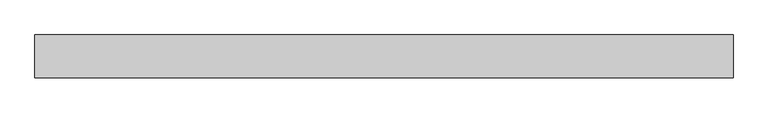
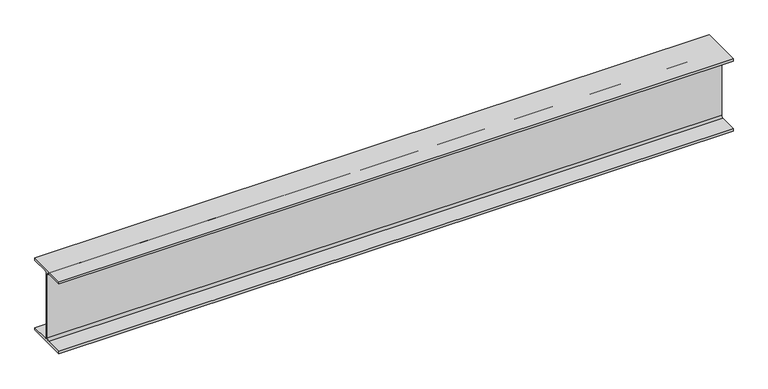
"""IFC4 building model written with IfcOpenShell, lengths in millimetres: beam geometry, Steel Beam_H-KSD3502 : H_SB_ASB_H-250x125x6x9."""

from ifc_helpers import new_model, si_unit, point, frame, frame_2d, origin, place, context, project, spatial, polyline, circle_curve, trimmed, segment, composite_curve, outline, extrude, source, transform, mapped, element, save


def beam_119fac50(model_context):
    return source(origin(), model_context, "Body", "SweptSolid", [
        extrude(outline(composite_curve([segment(polyline([(82.5, -141.5), (82.5, -151.7), (-82.5, -151.7), (-82.5, -141.5), (-11.9, -141.5)]), True, "CONTINUOUS"), segment(trimmed(circle_curve(frame_2d((-11.9, -132.6)), 8.9), [point((-11.9, -141.5))], [point((-3.0, -132.6))], True, "CARTESIAN"), True, "CONTINUOUS"), segment(polyline([(-3.0, -132.6), (-3.0, 132.6)]), True, "CONTINUOUS"), segment(trimmed(circle_curve(frame_2d((-11.9, 132.6)), 8.9), [point((-3.0, 132.6))], [point((-11.9, 141.5))], True, "CARTESIAN"), True, "CONTINUOUS"), segment(polyline([(-11.9, 141.5), (-82.5, 141.5), (-82.5, 151.7), (82.5, 151.7), (82.5, 141.5), (11.9, 141.5)]), True, "CONTINUOUS"), segment(trimmed(circle_curve(frame_2d((11.9, 132.6)), 8.9), [point((11.9, 141.5))], [point((3.0, 132.6))], True, "CARTESIAN"), True, "CONTINUOUS"), segment(polyline([(3.0, 132.6), (3.0, -132.6)]), True, "CONTINUOUS"), segment(trimmed(circle_curve(frame_2d((11.9, -132.6)), 8.9), [point((3.0, -132.6))], [point((11.9, -141.5))], True, "CARTESIAN"), True, "CONTINUOUS"), segment(polyline([(11.9, -141.5), (82.5, -141.5)]), True, "CONTINUOUS")], self_intersect=False)), frame((-1404.8000503, 0.0, 0.0), z_axis=(1.0, 0.0, 0.0), x_axis=(0.0, 1.0, 0.0)), (0.0, 0.0, 1.0), 2674.6999215),
    ])


if __name__ == "__main__":
    model = new_model("IFC4")
    model_context = context("Model", 3, world=origin())
    ifc_project = project(units=[si_unit("LENGTHUNIT", "METRE", prefix="MILLI")], contexts=[model_context])
    site = spatial("IfcSite", under=ifc_project)
    building = spatial("IfcBuilding", under=site)
    placement = place(None, origin())
    beam_shape = beam_119fac50(model_context)
    element("IfcBeam", 1, ObjectType="Steel Beam_H-KSD3502 : H_SB_ASB_H-250x125x6x9", at=placement, inside=building, context=model_context, shape_type="MappedRepresentation", body=[
        mapped(beam_shape, transform((0.0, 0.0, 0.0), x_axis=(1.0, 0.0, 0.0), y_axis=(0.0, 1.0, 0.0), z_axis=(0.0, 0.0, 1.0))),
    ])
    save(model, "model.ifc")

# Revit data of these elements
# Type "Steel Beam_H-KSD3502 : H_SB_ASB_H-250x125x6x9"
#   Width = 12.5 cm
#   Web Thickness = 0.6 cm
#   Web Fillet = 1.2 cm
#   Warping Constant = 42539.8 cm⁶
#   Torsional Moment of Inertia = 7.8102 cm⁴
#   Torsional Modulus = 1.0 cm³
#   Section Area = 37.66 cm²
#   Plastic Modulus weak axis = 73.1 cm³
#   Plastic Modulus strong axis = 366.0 cm³
#   Perimeter = 0.97 m²/m
#   Nominal Weight = 29.60 kgf/m
#   Moment of Inertia weak axis = 294.00 cm⁴
#   Moment of Inertia strong axis = 4050.00 cm⁴
#   Height = 25.0 cm
#   Flange Thickness = 0.9 cm
#   Elastic Modulus weak axis = 47.0 cm³
#   Elastic Modulus strong axis = 324.0 cm³
#   Centroid Vertical = 12.5 cm
#   Centroid Horizontal = 6.25 cm
#   Length [instance default] = 1.5240 m
#   Structural Material [instance default] = Steel, 45-345
#   Assembly Code = ""
# Element 1 (IfcBeam, "Steel Beam_H-KSD3502 : H_SB_ASB_H-250x125x6x9")
#   Structural Material = none
# Materials
#   "Steel, 45-345": class "Metal", colour RGB 189 187 185, transparency 0, Description = "Steel 345 MPa", Cost = 0
